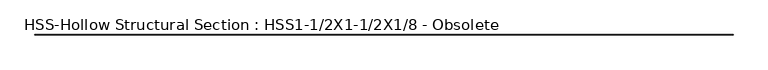
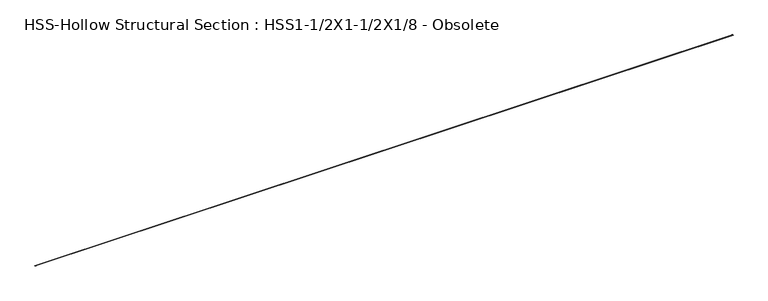
"""IFC4 building model written with IfcOpenShell, lengths in millimetres: beam geometry, HSS-Hollow Structural Section : HSS1-1/2X1-1/2X1/8 - Obsolete."""

from ifc_helpers import new_model, si_unit, point, frame, frame_2d, origin, place, context, project, spatial, polyline, circle_curve, trimmed, segment, composite_curve, outline, extrude, source, transform, mapped, element, save


def hss_hollow_structural_section_hss1_1_2x1_1_2x1_8_obsolete_ffed97b7(model_context):
    return source(origin(), model_context, "Body", "SweptSolid", [
        extrude(outline(composite_curve([segment(polyline([(19.05, 13.1572), (19.05, -13.1572)]), True, "CONTINUOUS"), segment(trimmed(circle_curve(frame_2d((13.1572, -13.1572)), 5.8928), [point((19.05, -13.1572))], [point((13.1572, -19.05))], False, "CARTESIAN"), True, "CONTINUOUS"), segment(polyline([(13.1572, -19.05), (-13.1572, -19.05)]), True, "CONTINUOUS"), segment(trimmed(circle_curve(frame_2d((-13.1572, -13.1572)), 5.8928), [point((-13.1572, -19.05))], [point((-19.05, -13.1572))], False, "CARTESIAN"), True, "CONTINUOUS"), segment(polyline([(-19.05, -13.1572), (-19.05, 13.1572)]), True, "CONTINUOUS"), segment(trimmed(circle_curve(frame_2d((-13.1572, 13.1572)), 5.8928), [point((-19.05, 13.1572))], [point((-13.1572, 19.05))], False, "CARTESIAN"), True, "CONTINUOUS"), segment(polyline([(-13.1572, 19.05), (13.1572, 19.05)]), True, "CONTINUOUS"), segment(trimmed(circle_curve(frame_2d((13.1572, 13.1572)), 5.8928), [point((13.1572, 19.05))], [point((19.05, 13.1572))], False, "CARTESIAN"), True, "CONTINUOUS")], self_intersect=False), holes=[composite_curve([segment(trimmed(circle_curve(frame_2d((-13.1572, 13.1572)), 2.9464), [point((-13.1572, 16.1036))], [point((-16.1036, 13.1572))], True, "CARTESIAN"), True, "CONTINUOUS"), segment(polyline([(-16.1036, 13.1572), (-16.1036, -13.1572)]), True, "CONTINUOUS"), segment(trimmed(circle_curve(frame_2d((-13.1572, -13.1572)), 2.9464), [point((-16.1036, -13.1572))], [point((-13.1572, -16.1036))], True, "CARTESIAN"), True, "CONTINUOUS"), segment(polyline([(-13.1572, -16.1036), (13.1572, -16.1036)]), True, "CONTINUOUS"), segment(trimmed(circle_curve(frame_2d((13.1572, -13.1572)), 2.9464), [point((13.1572, -16.1036))], [point((16.1036, -13.1572))], True, "CARTESIAN"), True, "CONTINUOUS"), segment(polyline([(16.1036, -13.1572), (16.1036, 13.1572)]), True, "CONTINUOUS"), segment(trimmed(circle_curve(frame_2d((13.1572, 13.1572)), 2.9464), [point((16.1036, 13.1572))], [point((13.1572, 16.1036))], True, "CARTESIAN"), True, "CONTINUOUS"), segment(polyline([(13.1572, 16.1036), (-13.1572, 16.1036)]), True, "CONTINUOUS")], self_intersect=False)]), frame((-44656.3750001, 0.0, 0.0), z_axis=(1.0, 0.0, 0.0), x_axis=(0.0, 1.0, 0.0)), (0.0, 0.0, 1.0), 89312.7500002),
    ])


if __name__ == "__main__":
    model = new_model("IFC4")
    model_context = context("Model", 3, world=origin())
    ifc_project = project(units=[si_unit("LENGTHUNIT", "METRE", prefix="MILLI")], contexts=[model_context])
    site = spatial("IfcSite", under=ifc_project)
    building = spatial("IfcBuilding", under=site)
    placement = place(None, origin())
    hss_hollow_structural_section_hss1_1_2x1_1_2x1_8_obsolete_shape = hss_hollow_structural_section_hss1_1_2x1_1_2x1_8_obsolete_ffed97b7(model_context)
    element("IfcBeam", 1, ObjectType="HSS-Hollow Structural Section : HSS1-1/2X1-1/2X1/8 - Obsolete", at=placement, inside=building, context=model_context, shape_type="MappedRepresentation", body=[
        mapped(hss_hollow_structural_section_hss1_1_2x1_1_2x1_8_obsolete_shape, transform((0.0, 0.0, 0.0), x_axis=(1.0, 0.0, 0.0), y_axis=(0.0, 1.0, 0.0), z_axis=(0.0, 0.0, 1.0))),
    ])
    save(model, "model.ifc")

# Revit data of these elements
# Type "HSS-Hollow Structural Section : HSS1-1/2X1-1/2X1/8 - Obsolete"
#   Assembly Code = "B10"
#   Shape = "Square"
#   W = 2.19
#   Ht = 0' - 1 1/2"
#   Length [instance default] = 5' - 0"
#   b = 0' - 1 1/2"
#   kr = 0' - 0.232"
#   t = 0' - 0.116"
#   A = 0.00423611 SF
#   Structural Material [instance default] = 1 1/2" X 1 1/2" x 1/8" ALUM. TUBE
# Element 1 (IfcBeam, "HSS-Hollow Structural Section : HSS1-1/2X1-1/2X1/8 - Obsolete")
#   Materials on its faces: "1 1/2\" X 1 1/2\" x 1/8\" ALUM. TUBE"
# Materials
#   "1 1/2\" X 1 1/2\" x 1/8\" ALUM. TUBE": class "Metal", colour RGB 199 199 199, transparency 0, Description = "Carbon steel", Cost = 0
